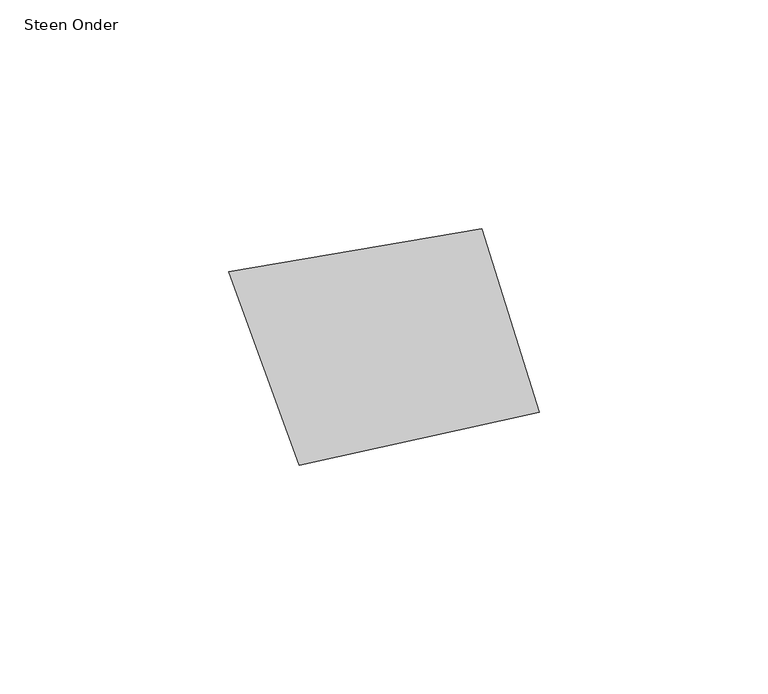
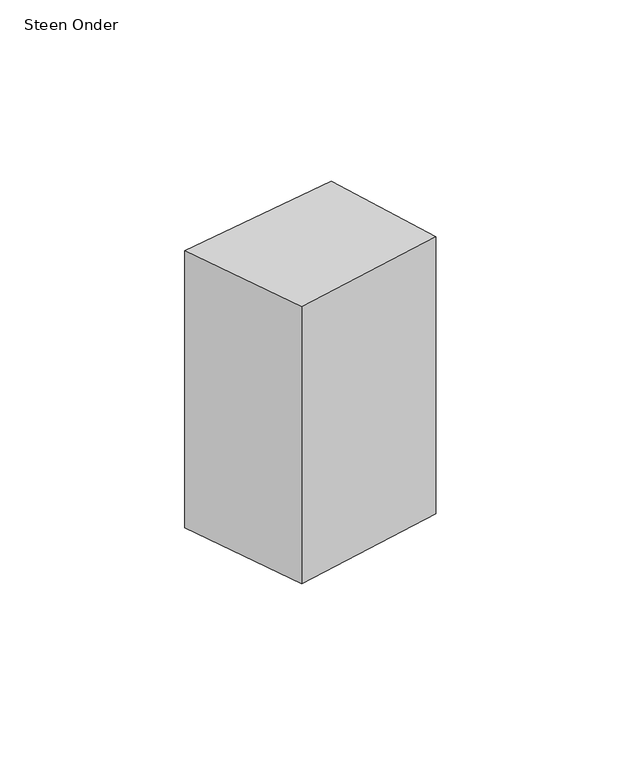
"""IFC4 building model written with IfcOpenShell, lengths in millimetres: proxy geometry, 00_GMA_steen_versie_4 : Steen Onder."""

from ifc_helpers import new_model, si_unit, origin, origin_with_axes, place, context, project, spatial, polyline, outline, extrude, source, transform, mapped, element, save


def steen_onder_99f9f282(model_context):
    return source(origin(), model_context, "Body", "SweptSolid", [
        extrude(outline(polyline([(95.0415986, 85.4929656), (107.6864014, 45.3564304), (55.2118589, 33.7844133), (39.7578472, 76.123298), (95.0415986, 85.4929656)])), origin_with_axes(), (0.0, 0.0, 1.0), 100.0),
    ])


if __name__ == "__main__":
    model = new_model("IFC4")
    model_context = context("Model", 3, world=origin())
    ifc_project = project(units=[si_unit("LENGTHUNIT", "METRE", prefix="MILLI")], contexts=[model_context])
    site = spatial("IfcSite", under=ifc_project)
    building = spatial("IfcBuilding", under=site)
    placement = place(None, origin())
    steen_onder_shape = steen_onder_99f9f282(model_context)
    element("IfcBuildingElementProxy", 1, Name="00_GMA_steen_versie_4 : Steen Onder", ObjectType="00_GMA_steen_versie_4 : Steen Onder", at=placement, inside=building, context=model_context, shape_type="MappedRepresentation", body=[
        mapped(steen_onder_shape, transform((0.0, 0.0, 0.0), x_axis=(1.0, 0.0, 0.0), y_axis=(0.0, 1.0, 0.0), z_axis=(0.0, 0.0, 1.0))),
    ])
    save(model, "model.ifc")

# Revit data of these elements
# Type "00_GMA_steen_versie_4 : Steen Onder"
#   StootVoegHalfBoven [instance default] = 5 mm
#   StootVoegHalf [instance default] = 5 mm
#   StootVoegBreedteOnder = 10 mm
#   StootVoegBreedteBoven = 10 mm
#   Steendikte = 100 mm
#   LintVoegOnderHalf = 0 mm
#   LintVoegOnder = 0 mm
#   LintVoegBovenHalf = 5 mm
#   LintVoegBoven = 10 mm
#   materiaal = none
#   MateriaalVoeg = none
#   Default Elevation = 0
